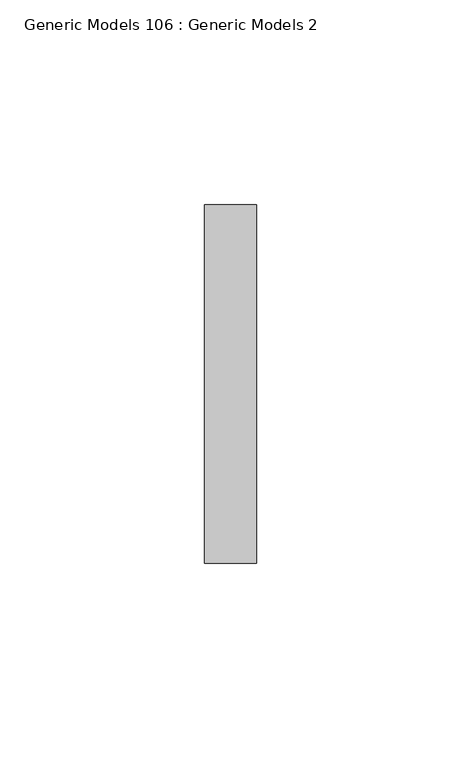
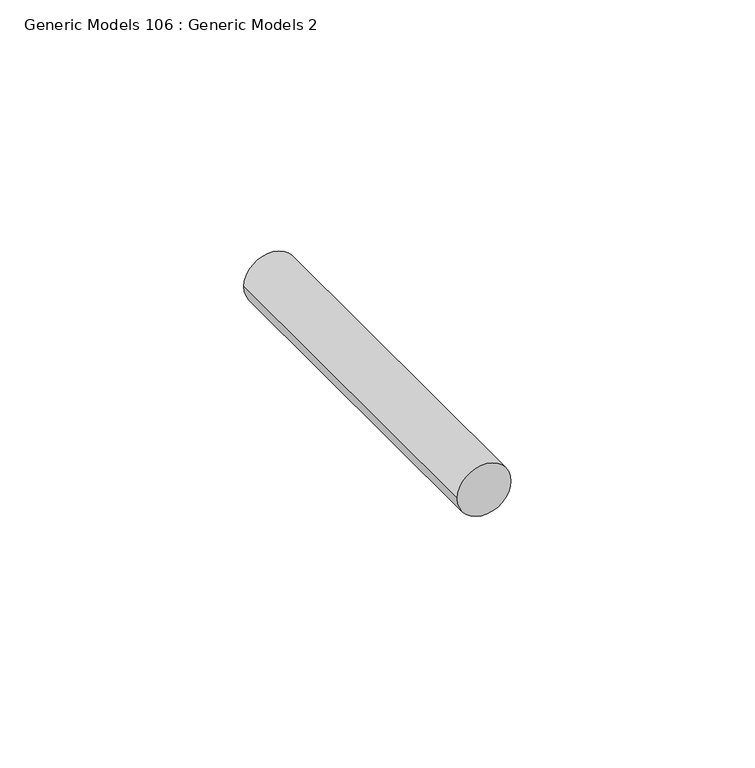
"""IFC4 building model written with IfcOpenShell, lengths in millimetres: proxy geometry, Generic Models 106 : Generic Models 2."""

from ifc_helpers import new_model, si_unit, point, frame, frame_2d, origin, place, context, project, spatial, circle_curve, trimmed, segment, composite_curve, outline, extrude, source, transform, mapped, element, save


def generic_models_106_generic_models_2_e5d8eed9(model_context):
    return source(origin(), model_context, "Body", "SweptSolid", [
        extrude(outline(composite_curve([segment(trimmed(circle_curve(frame_2d((37517.3905034, 6289.9828124)), 6.35), [point((37517.3905034, 6283.6328124))], [point((37517.3905034, 6296.3328124))], False, "CARTESIAN"), True, "CONTINUOUS"), segment(trimmed(circle_curve(frame_2d((37517.3905034, 6289.9828124)), 6.35), [point((37517.3905034, 6296.3328124))], [point((37517.3905034, 6283.6328124))], False, "CARTESIAN"), True, "CONTINUOUS")], self_intersect=False)), frame((0.0, 1848.3666731, 0.0), z_axis=(0.0, 1.0, 0.0), x_axis=(0.0, 0.0, 1.0)), (0.0, 0.0, 1.0), 87.551022),
    ])


if __name__ == "__main__":
    model = new_model("IFC4")
    model_context = context("Model", 3, world=origin())
    ifc_project = project(units=[si_unit("LENGTHUNIT", "METRE", prefix="MILLI")], contexts=[model_context])
    site = spatial("IfcSite", under=ifc_project)
    building = spatial("IfcBuilding", under=site)
    placement = place(None, origin())
    generic_models_106_generic_models_2_shape = generic_models_106_generic_models_2_e5d8eed9(model_context)
    element("IfcBuildingElementProxy", 1, Name="Generic Models 106 : Generic Models 2", ObjectType="Generic Models 106 : Generic Models 2", at=placement, inside=building, context=model_context, shape_type="MappedRepresentation", body=[
        mapped(generic_models_106_generic_models_2_shape, transform((0.0, 0.0, 0.0), x_axis=(1.0, 0.0, 0.0), y_axis=(0.0, 1.0, 0.0), z_axis=(0.0, 0.0, 1.0))),
    ])
    save(model, "model.ifc")

# Revit data of these elements
# Element 1 (IfcBuildingElementProxy, "Generic Models 106 : Generic Models 2")
#   Materials on its faces: "S.S. LAG BOLT - SEE STRUCT. DWGS"
# Materials
#   "S.S. LAG BOLT - SEE STRUCT. DWGS": class "Generic", colour RGB 120 120 120, transparency 0, Cost = 0
